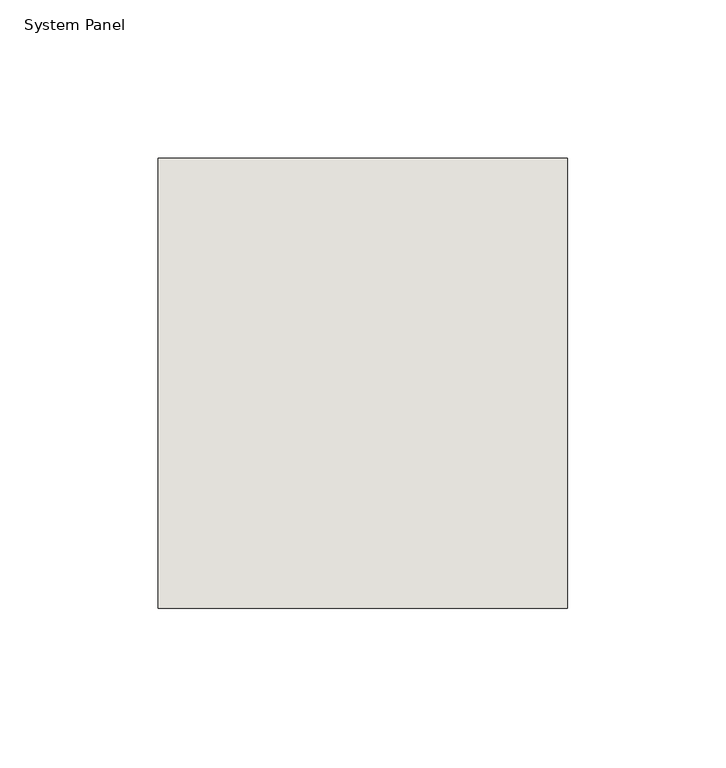
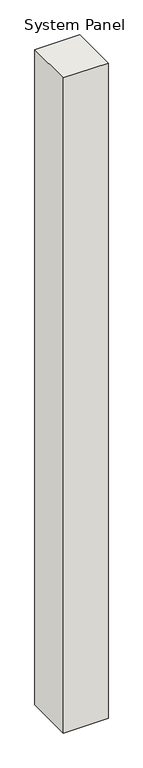
"""IFC4 building model written with IfcOpenShell, lengths in millimetres: wall geometry, System Panel : NLRS_21_CWP_hsb-vulling minerale wol 142 _gen_rsf."""

import ifcopenshell
import ifcopenshell.guid

model = None  # the IFC model being written
_history = None  # IfcOwnerHistory: only IFC2X3 demands one
_inside = {}  # id of a spatial element -> (the spatial element, [elements in it])
_under = {}  # id of a project, library or spatial element -> (it, [spatial elements below it])
_declared = {}  # id of a project -> (the project, [libraries it declares])
_typed = {}  # id of a type object -> (the type object, [elements of that type])
_made_of = {}  # id of a material, layer set ... -> (it, [elements and type objects made of it])


def new_model(schema):
    """Start an empty IFC model of exactly this schema.

    Asked for "IFC4X3", IfcOpenShell would pick the latest addendum, in which some entities
    have other attributes; the version numbers below select the first issue.
    IFC2X3 requires an IfcOwnerHistory on every rooted entity: one is made here for all.
    """
    global model, _history
    if schema == "IFC4X3":
        model = ifcopenshell.file(schema_version=(4, 3, 0, 0))
    else:
        model = ifcopenshell.file(schema=schema)
    _inside.clear()
    _under.clear()
    _declared.clear()
    _typed.clear()
    _made_of.clear()
    _history = None
    if model.schema == "IFC2X3":
        org = make("IfcOrganization", Name="unknown")
        user = make(
            "IfcPersonAndOrganization",
            ThePerson=make("IfcPerson", FamilyName="unknown"),
            TheOrganization=org,
        )
        app = make(
            "IfcApplication",
            ApplicationDeveloper=org,
            Version="unknown",
            ApplicationFullName="unknown",
            ApplicationIdentifier="unknown",
        )
        _history = make(
            "IfcOwnerHistory",
            OwningUser=user,
            OwningApplication=app,
            ChangeAction="ADDED",
            CreationDate=0,
        )
    return model


def make(cls, **values):
    """One entity of the class cls with the attributes given. An attribute that is None is left unset."""
    return model.create_entity(
        cls, **{name: value for name, value in values.items() if value is not None}
    )


def rooted(cls, **values):
    """An entity with a GlobalId (a new one), such as an element, a storey or a relation."""
    return make(cls, GlobalId=ifcopenshell.guid.new(), OwnerHistory=_history, **values)


def si_unit(unit_type, name, prefix=None):
    """IfcSIUnit, for example si_unit("LENGTHUNIT", "METRE", prefix="MILLI")."""
    return make("IfcSIUnit", UnitType=unit_type, Prefix=prefix, Name=name)


def assignment(units):
    """IfcUnitAssignment: the units of a project."""
    return None if units is None else make("IfcUnitAssignment", Units=units)


def point(xyz):
    """IfcCartesianPoint."""
    return None if xyz is None else make("IfcCartesianPoint", Coordinates=xyz)


def direction(xyz):
    """IfcDirection."""
    return None if xyz is None else make("IfcDirection", DirectionRatios=xyz)


def frame(location, z_axis=None, x_axis=None):
    """IfcAxis2Placement3D, a coordinate frame: its origin and axes. An axis left out is left unset."""
    return make(
        "IfcAxis2Placement3D",
        Location=point(location),
        Axis=direction(z_axis),
        RefDirection=direction(x_axis),
    )


def origin():
    """The frame at (0, 0, 0) with its axes left unset."""
    return frame((0.0, 0.0, 0.0))


def origin_with_axes():
    """The frame at (0, 0, 0) with the z axis (0, 0, 1) and the x axis (1, 0, 0) written out."""
    return frame((0.0, 0.0, 0.0), z_axis=(0.0, 0.0, 1.0), x_axis=(1.0, 0.0, 0.0))


def place(relative_to, where):
    """IfcLocalPlacement: puts the frame where relative to a parent placement (None: the world)."""
    return make(
        "IfcLocalPlacement", PlacementRelTo=relative_to, RelativePlacement=where
    )


def context(
    kind, dimensions, precision=None, world=None, true_north=None, identifier=None
):
    """IfcGeometricRepresentationContext, for example the 3D "Model" context."""
    return make(
        "IfcGeometricRepresentationContext",
        ContextIdentifier=identifier,
        ContextType=kind,
        CoordinateSpaceDimension=dimensions,
        Precision=precision,
        WorldCoordinateSystem=world,
        TrueNorth=true_north,
    )


def project(units=None, contexts=None):
    """IfcProject with its units and contexts."""
    return rooted(
        "IfcProject",
        Name="project",
        RepresentationContexts=contexts,
        UnitsInContext=assignment(units),
    )


def spatial(cls, under=None, at=None, **own):
    """A site, building, storey or space (cls), placed at a placement, below another one or the project."""
    s = rooted(cls, ObjectPlacement=at, **own)
    if under is not None:
        _under.setdefault(under.id(), (under, []))[1].append(s)
    return s


def polyline(points):
    """IfcPolyline through the points."""
    return make("IfcPolyline", Points=[point(p) for p in points])


def outline(outer, holes=None, kind="AREA"):
    """IfcArbitraryClosedProfileDef: a profile drawn as a closed curve; with holes, ...WithVoids."""
    if holes is None:
        return make("IfcArbitraryClosedProfileDef", ProfileType=kind, OuterCurve=outer)
    return make(
        "IfcArbitraryProfileDefWithVoids",
        ProfileType=kind,
        OuterCurve=outer,
        InnerCurves=holes,
    )


def extrude(swept, where, along, depth):
    """IfcExtrudedAreaSolid: the profile swept, set in the frame where, extruded along a direction by depth."""
    return make(
        "IfcExtrudedAreaSolid",
        SweptArea=swept,
        Position=where,
        ExtrudedDirection=direction(along),
        Depth=depth,
    )


def shape(context_of_items, identifier, shape_type, items):
    """IfcShapeRepresentation: the items that make up one representation, for example the "Body"."""
    return make(
        "IfcShapeRepresentation",
        ContextOfItems=context_of_items,
        RepresentationIdentifier=identifier,
        RepresentationType=shape_type,
        Items=items,
    )


def source(mapping_origin, context_of_items, identifier, shape_type, items):
    """IfcRepresentationMap: a shape defined once, which mapped items show again and again."""
    return make(
        "IfcRepresentationMap",
        MappingOrigin=mapping_origin,
        MappedRepresentation=shape(context_of_items, identifier, shape_type, items),
    )


def transform(
    local_origin,
    x_axis=None,
    y_axis=None,
    z_axis=None,
    scale=None,
    scale2=None,
    scale3=None,
    uniform=True,
):
    """IfcCartesianTransformationOperator3D, or its non-uniform kind. x_axis, y_axis, z_axis: its Axis1, 2, 3."""
    if uniform:
        return make(
            "IfcCartesianTransformationOperator3D",
            Axis1=direction(x_axis),
            Axis2=direction(y_axis),
            LocalOrigin=point(local_origin),
            Scale=scale,
            Axis3=direction(z_axis),
        )
    return make(
        "IfcCartesianTransformationOperator3DnonUniform",
        Axis1=direction(x_axis),
        Axis2=direction(y_axis),
        LocalOrigin=point(local_origin),
        Scale=scale,
        Axis3=direction(z_axis),
        Scale2=scale2,
        Scale3=scale3,
    )


def mapped(mapping_source, mapping_target):
    """IfcMappedItem: shows the shape of a source again, moved by a transform."""
    return make(
        "IfcMappedItem", MappingSource=mapping_source, MappingTarget=mapping_target
    )


def made_of(thing, what):
    """Note that an element or type object is made of a material, layer set ...; save() writes the relation."""
    if what is not None:
        _made_of.setdefault(what.id(), (what, []))[1].append(thing)
    return thing


def element(
    cls,
    number,
    at=None,
    inside=None,
    cuts=None,
    type_object=None,
    material=None,
    context=None,
    identifier="Body",
    shape_type=None,
    held_by="IfcProductDefinitionShape",
    body=None,
    shapes=None,
    **own,
):
    """One element of the class cls, such as IfcWall. Its Tag is "e" and its number.

    at: its placement. inside: the storey or other place that contains it. cuts: it is an
    opening in that element (IfcRelVoidsElement). A single representation is given by context,
    identifier, shape_type and body (its items); several are given by shapes. held_by: the class
    of the entity that holds the representations. save() writes the other relations.
    """
    e = rooted(cls, Tag="e%d" % number, ObjectPlacement=at, **own)
    if body is not None:
        shapes = [shape(context, identifier, shape_type, body)]
    if shapes is not None:
        e.Representation = make(held_by, Representations=shapes)
    if inside is not None:
        _inside.setdefault(inside.id(), (inside, []))[1].append(e)
    if cuts is not None:
        rooted(
            "IfcRelVoidsElement", RelatingBuildingElement=cuts, RelatedOpeningElement=e
        )
    if type_object is not None:
        _typed.setdefault(type_object.id(), (type_object, []))[1].append(e)
    return made_of(e, material)


def aggregate(whole, parts):
    """IfcRelAggregates: a whole, such as a stair, and the parts it consists of."""
    return rooted("IfcRelAggregates", RelatingObject=whole, RelatedObjects=parts)


def save(model, path):
    """Write the relations noted so far, then the file.

    IfcRelAggregates (storeys below a building ...), IfcRelContainedInSpatialStructure (elements
    in a storey), IfcRelDefinesByType, IfcRelAssociatesMaterial and IfcRelDeclares: one each for
    every whole, place, type object, material and project.
    """
    for whole, parts in _under.values():
        aggregate(whole, parts)
    for where, things in _inside.values():
        rooted(
            "IfcRelContainedInSpatialStructure",
            RelatedElements=things,
            RelatingStructure=where,
        )
    for kind, things in _typed.values():
        rooted("IfcRelDefinesByType", RelatedObjects=things, RelatingType=kind)
    for what, things in _made_of.values():
        rooted("IfcRelAssociatesMaterial", RelatedObjects=things, RelatingMaterial=what)
    for by, libraries in _declared.values():
        rooted("IfcRelDeclares", RelatingContext=by, RelatedDefinitions=libraries)
    model.write(path)


def system_panel_6860f7c2(model_context):
    return source(origin(), model_context, "Body", "SweptSolid", [
        extrude(outline(polyline([(64.577947, -71.0), (-64.577947, -71.0), (-64.577947, 71.0), (64.577947, 71.0), (64.577947, -71.0)])), origin_with_axes(), (0.0, 0.0, 1.0), 2000.0),
    ])


if __name__ == "__main__":
    model = new_model("IFC4")
    model_context = context("Model", 3, world=origin())
    ifc_project = project(units=[si_unit("LENGTHUNIT", "METRE", prefix="MILLI")], contexts=[model_context])
    site = spatial("IfcSite", under=ifc_project)
    building = spatial("IfcBuilding", under=site)
    placement = place(None, origin())
    system_panel_shape = system_panel_6860f7c2(model_context)
    element("IfcWall", 1, ObjectType="System Panel : NLRS_21_CWP_hsb-vulling minerale wol 142 _gen_rsf", at=placement, inside=building, context=model_context, shape_type="MappedRepresentation", body=[
        mapped(system_panel_shape, transform((0.0, 0.0, 0.0), x_axis=(1.0, 0.0, 0.0), y_axis=(0.0, 1.0, 0.0), z_axis=(0.0, 0.0, 1.0))),
    ])
    save(model, "model.ifc")

# Revit data of these elements
# Type "System Panel : NLRS_21_CWP_hsb-vulling minerale wol 142 _gen_rsf"
#   Type IfcGUID = "07M7mRoiH1CR8m_RSKIwpC"
#   Assembly Code = "21.23"
#   IfcExportAs = "IfcWall"
# Element 1 (IfcWall, "System Panel : NLRS_21_CWP_hsb-vulling minerale wol 142 _gen_rsf")
#   Materials on its faces: "NLRS_m1_isolatie minerale wol_gen_rsf"
# Materials
#   "NLRS_m1_isolatie minerale wol_gen_rsf": class "M - Anorganische materialen", colour RGB 200 200 140, transparency 0, Keynote = "m1", Manufacturer = "Revit Standards Foundation", URL = "www.revitstandards.org", Description = "isolatie minerale wol", Cost = 0
